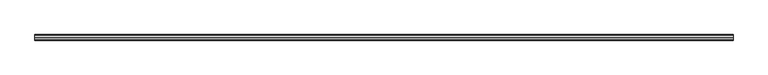
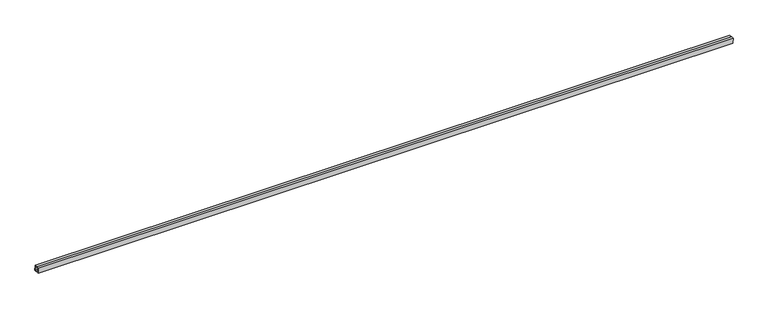
"""IFC4 building model written with IfcOpenShell, lengths in millimetres: proxy geometry, Inner panel:Inner panel:1:Inner panel:1 : Inner panel:Inner panel:300324:2:Inner panel:1:Inner panel:1 : Inner panel:Inner panel:300324:2 : Inner panel:Inner panel:1:Inner panel:1 : Inner panel:Inner panel:300324:300043:12 : Inner panel:Inner panel:1:Inner panel:1 : Inner panel:Inner panel:300324:2:Inner panel:1:Inner panel:1 : Inner panel:Inner panel:300324:2 : Inner panel:Inner panel:1:Inner panel:1 : Inner panel:Inner panel:300324:300043:308120."""

import ifcopenshell
import ifcopenshell.guid

model = None  # the IFC model being written
_history = None  # IfcOwnerHistory: only IFC2X3 demands one
_inside = {}  # id of a spatial element -> (the spatial element, [elements in it])
_under = {}  # id of a project, library or spatial element -> (it, [spatial elements below it])
_declared = {}  # id of a project -> (the project, [libraries it declares])
_typed = {}  # id of a type object -> (the type object, [elements of that type])
_made_of = {}  # id of a material, layer set ... -> (it, [elements and type objects made of it])


def new_model(schema):
    """Start an empty IFC model of exactly this schema.

    Asked for "IFC4X3", IfcOpenShell would pick the latest addendum, in which some entities
    have other attributes; the version numbers below select the first issue.
    IFC2X3 requires an IfcOwnerHistory on every rooted entity: one is made here for all.
    """
    global model, _history
    if schema == "IFC4X3":
        model = ifcopenshell.file(schema_version=(4, 3, 0, 0))
    else:
        model = ifcopenshell.file(schema=schema)
    _inside.clear()
    _under.clear()
    _declared.clear()
    _typed.clear()
    _made_of.clear()
    _history = None
    if model.schema == "IFC2X3":
        org = make("IfcOrganization", Name="unknown")
        user = make(
            "IfcPersonAndOrganization",
            ThePerson=make("IfcPerson", FamilyName="unknown"),
            TheOrganization=org,
        )
        app = make(
            "IfcApplication",
            ApplicationDeveloper=org,
            Version="unknown",
            ApplicationFullName="unknown",
            ApplicationIdentifier="unknown",
        )
        _history = make(
            "IfcOwnerHistory",
            OwningUser=user,
            OwningApplication=app,
            ChangeAction="ADDED",
            CreationDate=0,
        )
    return model


def make(cls, **values):
    """One entity of the class cls with the attributes given. An attribute that is None is left unset."""
    return model.create_entity(
        cls, **{name: value for name, value in values.items() if value is not None}
    )


def rooted(cls, **values):
    """An entity with a GlobalId (a new one), such as an element, a storey or a relation."""
    return make(cls, GlobalId=ifcopenshell.guid.new(), OwnerHistory=_history, **values)


def si_unit(unit_type, name, prefix=None):
    """IfcSIUnit, for example si_unit("LENGTHUNIT", "METRE", prefix="MILLI")."""
    return make("IfcSIUnit", UnitType=unit_type, Prefix=prefix, Name=name)


def assignment(units):
    """IfcUnitAssignment: the units of a project."""
    return None if units is None else make("IfcUnitAssignment", Units=units)


def point(xyz):
    """IfcCartesianPoint."""
    return None if xyz is None else make("IfcCartesianPoint", Coordinates=xyz)


def direction(xyz):
    """IfcDirection."""
    return None if xyz is None else make("IfcDirection", DirectionRatios=xyz)


def frame(location, z_axis=None, x_axis=None):
    """IfcAxis2Placement3D, a coordinate frame: its origin and axes. An axis left out is left unset."""
    return make(
        "IfcAxis2Placement3D",
        Location=point(location),
        Axis=direction(z_axis),
        RefDirection=direction(x_axis),
    )


def origin():
    """The frame at (0, 0, 0) with its axes left unset."""
    return frame((0.0, 0.0, 0.0))


def place(relative_to, where):
    """IfcLocalPlacement: puts the frame where relative to a parent placement (None: the world)."""
    return make(
        "IfcLocalPlacement", PlacementRelTo=relative_to, RelativePlacement=where
    )


def context(
    kind, dimensions, precision=None, world=None, true_north=None, identifier=None
):
    """IfcGeometricRepresentationContext, for example the 3D "Model" context."""
    return make(
        "IfcGeometricRepresentationContext",
        ContextIdentifier=identifier,
        ContextType=kind,
        CoordinateSpaceDimension=dimensions,
        Precision=precision,
        WorldCoordinateSystem=world,
        TrueNorth=true_north,
    )


def project(units=None, contexts=None):
    """IfcProject with its units and contexts."""
    return rooted(
        "IfcProject",
        Name="project",
        RepresentationContexts=contexts,
        UnitsInContext=assignment(units),
    )


def spatial(cls, under=None, at=None, **own):
    """A site, building, storey or space (cls), placed at a placement, below another one or the project."""
    s = rooted(cls, ObjectPlacement=at, **own)
    if under is not None:
        _under.setdefault(under.id(), (under, []))[1].append(s)
    return s


def polyline(points):
    """IfcPolyline through the points."""
    return make("IfcPolyline", Points=[point(p) for p in points])


def outline(outer, holes=None, kind="AREA"):
    """IfcArbitraryClosedProfileDef: a profile drawn as a closed curve; with holes, ...WithVoids."""
    if holes is None:
        return make("IfcArbitraryClosedProfileDef", ProfileType=kind, OuterCurve=outer)
    return make(
        "IfcArbitraryProfileDefWithVoids",
        ProfileType=kind,
        OuterCurve=outer,
        InnerCurves=holes,
    )


def extrude(swept, where, along, depth):
    """IfcExtrudedAreaSolid: the profile swept, set in the frame where, extruded along a direction by depth."""
    return make(
        "IfcExtrudedAreaSolid",
        SweptArea=swept,
        Position=where,
        ExtrudedDirection=direction(along),
        Depth=depth,
    )


def shape(context_of_items, identifier, shape_type, items):
    """IfcShapeRepresentation: the items that make up one representation, for example the "Body"."""
    return make(
        "IfcShapeRepresentation",
        ContextOfItems=context_of_items,
        RepresentationIdentifier=identifier,
        RepresentationType=shape_type,
        Items=items,
    )


def source(mapping_origin, context_of_items, identifier, shape_type, items):
    """IfcRepresentationMap: a shape defined once, which mapped items show again and again."""
    return make(
        "IfcRepresentationMap",
        MappingOrigin=mapping_origin,
        MappedRepresentation=shape(context_of_items, identifier, shape_type, items),
    )


def transform(
    local_origin,
    x_axis=None,
    y_axis=None,
    z_axis=None,
    scale=None,
    scale2=None,
    scale3=None,
    uniform=True,
):
    """IfcCartesianTransformationOperator3D, or its non-uniform kind. x_axis, y_axis, z_axis: its Axis1, 2, 3."""
    if uniform:
        return make(
            "IfcCartesianTransformationOperator3D",
            Axis1=direction(x_axis),
            Axis2=direction(y_axis),
            LocalOrigin=point(local_origin),
            Scale=scale,
            Axis3=direction(z_axis),
        )
    return make(
        "IfcCartesianTransformationOperator3DnonUniform",
        Axis1=direction(x_axis),
        Axis2=direction(y_axis),
        LocalOrigin=point(local_origin),
        Scale=scale,
        Axis3=direction(z_axis),
        Scale2=scale2,
        Scale3=scale3,
    )


def mapped(mapping_source, mapping_target):
    """IfcMappedItem: shows the shape of a source again, moved by a transform."""
    return make(
        "IfcMappedItem", MappingSource=mapping_source, MappingTarget=mapping_target
    )


def made_of(thing, what):
    """Note that an element or type object is made of a material, layer set ...; save() writes the relation."""
    if what is not None:
        _made_of.setdefault(what.id(), (what, []))[1].append(thing)
    return thing


def element(
    cls,
    number,
    at=None,
    inside=None,
    cuts=None,
    type_object=None,
    material=None,
    context=None,
    identifier="Body",
    shape_type=None,
    held_by="IfcProductDefinitionShape",
    body=None,
    shapes=None,
    **own,
):
    """One element of the class cls, such as IfcWall. Its Tag is "e" and its number.

    at: its placement. inside: the storey or other place that contains it. cuts: it is an
    opening in that element (IfcRelVoidsElement). A single representation is given by context,
    identifier, shape_type and body (its items); several are given by shapes. held_by: the class
    of the entity that holds the representations. save() writes the other relations.
    """
    e = rooted(cls, Tag="e%d" % number, ObjectPlacement=at, **own)
    if body is not None:
        shapes = [shape(context, identifier, shape_type, body)]
    if shapes is not None:
        e.Representation = make(held_by, Representations=shapes)
    if inside is not None:
        _inside.setdefault(inside.id(), (inside, []))[1].append(e)
    if cuts is not None:
        rooted(
            "IfcRelVoidsElement", RelatingBuildingElement=cuts, RelatedOpeningElement=e
        )
    if type_object is not None:
        _typed.setdefault(type_object.id(), (type_object, []))[1].append(e)
    return made_of(e, material)


def aggregate(whole, parts):
    """IfcRelAggregates: a whole, such as a stair, and the parts it consists of."""
    return rooted("IfcRelAggregates", RelatingObject=whole, RelatedObjects=parts)


def save(model, path):
    """Write the relations noted so far, then the file.

    IfcRelAggregates (storeys below a building ...), IfcRelContainedInSpatialStructure (elements
    in a storey), IfcRelDefinesByType, IfcRelAssociatesMaterial and IfcRelDeclares: one each for
    every whole, place, type object, material and project.
    """
    for whole, parts in _under.values():
        aggregate(whole, parts)
    for where, things in _inside.values():
        rooted(
            "IfcRelContainedInSpatialStructure",
            RelatedElements=things,
            RelatingStructure=where,
        )
    for kind, things in _typed.values():
        rooted("IfcRelDefinesByType", RelatedObjects=things, RelatingType=kind)
    for what, things in _made_of.values():
        rooted("IfcRelAssociatesMaterial", RelatedObjects=things, RelatingMaterial=what)
    for by, libraries in _declared.values():
        rooted("IfcRelDeclares", RelatingContext=by, RelatedDefinitions=libraries)
    model.write(path)


def generic_models_874b4a9b(model_context):
    return source(origin(), model_context, "Body", "SweptSolid", [
        extrude(outline(polyline([(-579878.6983883, 3913.3147263), (-579860.4579651, 3914.0747439), (-579858.8718413, 3876.0077738), (-579896.9388114, 3874.4216501), (-579898.5249352, 3912.4886201), (-579880.284512, 3913.2486378), (-579880.1853793, 3910.8694521), (-579896.0466168, 3910.2085672), (-579894.6587585, 3876.8999684), (-579861.3501597, 3878.2878267), (-579862.738018, 3911.5964255), (-579878.5992555, 3910.9355406), (-579878.6983883, 3913.3147263)])), frame((588245.3367239, 0.0, 0.0), z_axis=(1.0, 0.0, 0.0), x_axis=(0.0, 1.0, 0.0)), (0.0, 0.0, 1.0), 4876.8),
    ])


if __name__ == "__main__":
    model = new_model("IFC4")
    model_context = context("Model", 3, world=origin())
    ifc_project = project(units=[si_unit("LENGTHUNIT", "METRE", prefix="MILLI")], contexts=[model_context])
    site = spatial("IfcSite", under=ifc_project)
    building = spatial("IfcBuilding", under=site)
    placement = place(None, origin())
    generic_models_shape = generic_models_874b4a9b(model_context)
    element("IfcBuildingElementProxy", 1, Name="Inner panel:Inner panel:1:Inner panel:1 : Inner panel:Inner panel:300324:2:Inner panel:1:Inner panel:1 : Inner panel:Inner panel:300324:2 : Inner panel:Inner panel:1:Inner panel:1 : Inner panel:Inner panel:300324:300043:12 : Inner panel:Inner panel:1:Inner panel:1 : Inner panel:Inner panel:300324:2:Inner panel:1:Inner panel:1 : Inner panel:Inner panel:300324:2 : Inner panel:Inner panel:1:Inner panel:1 : Inner panel:Inner panel:300324:300043:308120", ObjectType="Inner panel:Inner panel:1:Inner panel:1 : Inner panel:Inner panel:300324:2:Inner panel:1:Inner panel:1 : Inner panel:Inner panel:300324:2 : Inner panel:Inner panel:1:Inner panel:1 : Inner panel:Inner panel:300324:300043:12 : Inner panel:Inner panel:1:Inner panel:1 : Inner panel:Inner panel:300324:2:Inner panel:1:Inner panel:1 : Inner panel:Inner panel:300324:2 : Inner panel:Inner panel:1:Inner panel:1 : Inner panel:Inner panel:300324:300043:308120", at=placement, inside=building, context=model_context, shape_type="MappedRepresentation", body=[
        mapped(generic_models_shape, transform((0.0, 0.0, 0.0), x_axis=(1.0, 0.0, 0.0), y_axis=(0.0, 1.0, 0.0), z_axis=(0.0, 0.0, 1.0))),
    ])
    save(model, "model.ifc")

# Revit data of these elements
# Type "Inner panel:Inner panel:1:Inner panel:1 : Inner panel:Inner panel:300324:2:Inner panel:1:Inner panel:1 : Inner panel:Inner panel:300324:2 : Inner panel:Inner panel:1:Inner panel:1 : Inner panel:Inner panel:300324:300043:12 : Inner panel:Inner panel:1:Inner panel:1 : Inner panel:Inner panel:300324:2:Inner panel:1:Inner panel:1 : Inner panel:Inner panel:300324:2 : Inner panel:Inner panel:1:Inner panel:1 : Inner panel:Inner panel:300324:300043:308120"
#   NameOverride = "Inner panel:Inner panel:1:Inner panel:1 : Inner panel:Inner panel:300324:2:Inner panel:1:Inner panel:1 : Inner panel:Inner panel:300324:2 : Inner panel:Inner panel:1:Inner panel:1 : Inner panel:Inner panel:300324:300043:308120"
#   ObjectTypeOverride = "Inner panel:1:Inner panel:1 : Inner panel:Inner panel:300324:2 : Inner panel:Inner panel:1:Inner panel:1 : Inner panel:Inner panel:300324:300043"
#   Reference = "Inner panel"
#   Tag = "308120"
# Element 1 (IfcBuildingElementProxy, "Inner panel:Inner panel:1:Inner panel:1 : Inner panel:Inner panel:300324:2:Inner panel:1:Inner panel:1 : Inner panel:Inner panel:300324:2 : Inner panel:Inner panel:1:Inner panel:1 : Inner panel:Inner panel:300324:300043:12 : Inner panel:Inner panel:1:Inner panel:1 : Inner panel:Inner panel:300324:2:Inner panel:1:Inner panel:1 : Inner panel:Inner panel:300324:2 : Inner panel:Inner panel:1:Inner panel:1 : Inner panel:Inner panel:300324:300043:308120")
#   Materials on its faces: "1 1/2\" X 1 1/2\" SPLIT-SEAM SQUARE TUBING (~24\" CANTILEVER FROM C.L. OF GLULAM)"
# Materials
#   "1 1/2\" X 1 1/2\" SPLIT-SEAM SQUARE TUBING (~24\" CANTILEVER FROM C.L. OF GLULAM)": class "Unassigned", colour RGB 202 201 200, transparency 0, Cost = 0
